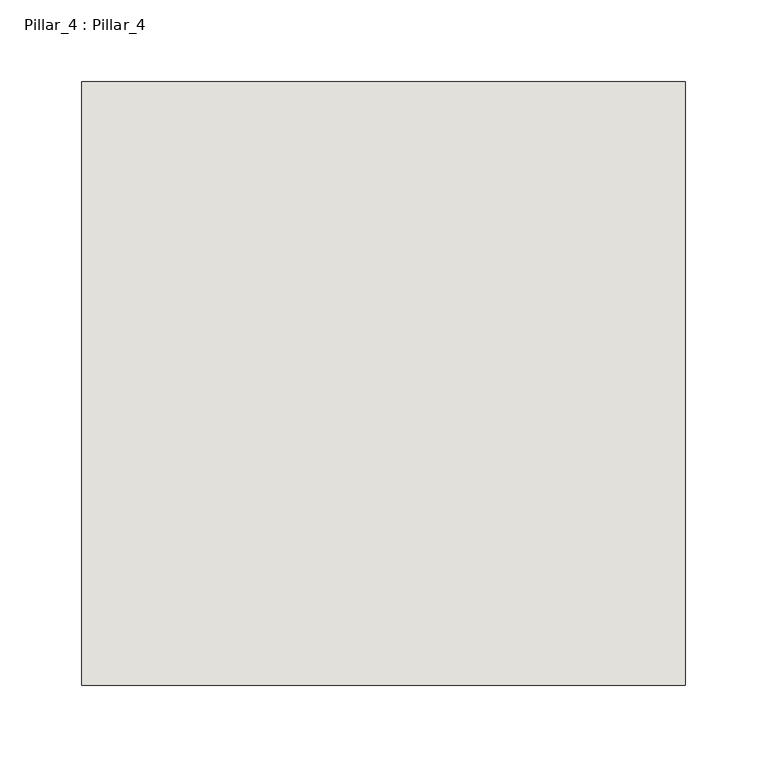
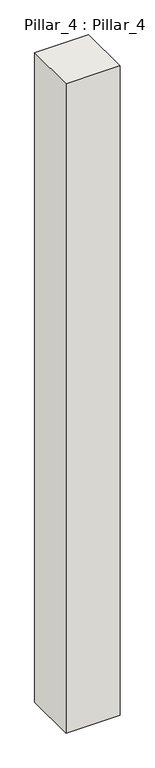
"""IFC4 building model written with IfcOpenShell, lengths in millimetres: wall geometry, Pillar_4 : Pillar_4."""

from ifc_helpers import new_model, si_unit, origin, origin_with_axes, place, context, project, spatial, polyline, outline, extrude, source, transform, mapped, element, save


def pillar_4_pillar_4_1424975a(model_context):
    return source(origin(), model_context, "Body", "SweptSolid", [
        extrude(outline(polyline([(235.0, 11970.0), (-135.0, 11970.0), (-135.0, 12340.0), (235.0, 12340.0), (235.0, 11970.0)])), origin_with_axes(), (0.0, 0.0, 1.0), 4700.0),
    ])


if __name__ == "__main__":
    model = new_model("IFC4")
    model_context = context("Model", 3, world=origin())
    ifc_project = project(units=[si_unit("LENGTHUNIT", "METRE", prefix="MILLI")], contexts=[model_context])
    site = spatial("IfcSite", under=ifc_project)
    building = spatial("IfcBuilding", under=site)
    placement = place(None, origin())
    pillar_4_pillar_4_shape = pillar_4_pillar_4_1424975a(model_context)
    element("IfcWall", 1, ObjectType="Pillar_4 : Pillar_4", at=placement, inside=building, context=model_context, shape_type="MappedRepresentation", body=[
        mapped(pillar_4_pillar_4_shape, transform((0.0, 0.0, 0.0), x_axis=(1.0, 0.0, 0.0), y_axis=(0.0, 1.0, 0.0), z_axis=(0.0, 0.0, 1.0))),
    ])
    save(model, "model.ifc")

# Revit data of these elements
# Type "Pillar_4 : Pillar_4"
#   NameOverride = "Pillar_4"
# Element 1 (IfcWall, "Pillar_4 : Pillar_4")
#   Materials on its faces: "IfcSurfaceStyle #33"
# Materials
#   "IfcSurfaceStyle #33": class "Unassigned", colour RGB 214 214 214, transparency 0
